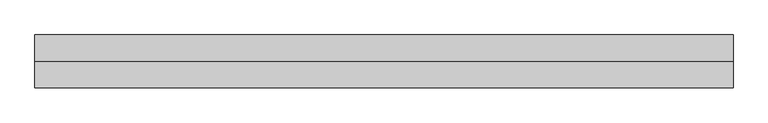
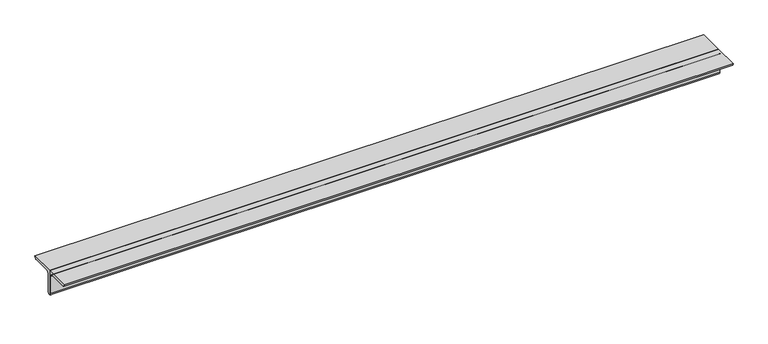
"""IFC4 building model written with IfcOpenShell, lengths in millimetres: member geometry, 0123_Steel Framing_2Ls-KSD3502 : H_SB_AR_S03_2Ls-130x130x12_HBR4."""

import ifcopenshell
import ifcopenshell.guid

model = None  # the IFC model being written
_history = None  # IfcOwnerHistory: only IFC2X3 demands one
_inside = {}  # id of a spatial element -> (the spatial element, [elements in it])
_under = {}  # id of a project, library or spatial element -> (it, [spatial elements below it])
_declared = {}  # id of a project -> (the project, [libraries it declares])
_typed = {}  # id of a type object -> (the type object, [elements of that type])
_made_of = {}  # id of a material, layer set ... -> (it, [elements and type objects made of it])


def new_model(schema):
    """Start an empty IFC model of exactly this schema.

    Asked for "IFC4X3", IfcOpenShell would pick the latest addendum, in which some entities
    have other attributes; the version numbers below select the first issue.
    IFC2X3 requires an IfcOwnerHistory on every rooted entity: one is made here for all.
    """
    global model, _history
    if schema == "IFC4X3":
        model = ifcopenshell.file(schema_version=(4, 3, 0, 0))
    else:
        model = ifcopenshell.file(schema=schema)
    _inside.clear()
    _under.clear()
    _declared.clear()
    _typed.clear()
    _made_of.clear()
    _history = None
    if model.schema == "IFC2X3":
        org = make("IfcOrganization", Name="unknown")
        user = make(
            "IfcPersonAndOrganization",
            ThePerson=make("IfcPerson", FamilyName="unknown"),
            TheOrganization=org,
        )
        app = make(
            "IfcApplication",
            ApplicationDeveloper=org,
            Version="unknown",
            ApplicationFullName="unknown",
            ApplicationIdentifier="unknown",
        )
        _history = make(
            "IfcOwnerHistory",
            OwningUser=user,
            OwningApplication=app,
            ChangeAction="ADDED",
            CreationDate=0,
        )
    return model


def make(cls, **values):
    """One entity of the class cls with the attributes given. An attribute that is None is left unset."""
    return model.create_entity(
        cls, **{name: value for name, value in values.items() if value is not None}
    )


def rooted(cls, **values):
    """An entity with a GlobalId (a new one), such as an element, a storey or a relation."""
    return make(cls, GlobalId=ifcopenshell.guid.new(), OwnerHistory=_history, **values)


def si_unit(unit_type, name, prefix=None):
    """IfcSIUnit, for example si_unit("LENGTHUNIT", "METRE", prefix="MILLI")."""
    return make("IfcSIUnit", UnitType=unit_type, Prefix=prefix, Name=name)


def assignment(units):
    """IfcUnitAssignment: the units of a project."""
    return None if units is None else make("IfcUnitAssignment", Units=units)


def point(xyz):
    """IfcCartesianPoint."""
    return None if xyz is None else make("IfcCartesianPoint", Coordinates=xyz)


def direction(xyz):
    """IfcDirection."""
    return None if xyz is None else make("IfcDirection", DirectionRatios=xyz)


def frame(location, z_axis=None, x_axis=None):
    """IfcAxis2Placement3D, a coordinate frame: its origin and axes. An axis left out is left unset."""
    return make(
        "IfcAxis2Placement3D",
        Location=point(location),
        Axis=direction(z_axis),
        RefDirection=direction(x_axis),
    )


def frame_2d(location, x_axis=None):
    """IfcAxis2Placement2D, a coordinate frame in the plane: its origin and x axis."""
    return make(
        "IfcAxis2Placement2D", Location=point(location), RefDirection=direction(x_axis)
    )


def origin():
    """The frame at (0, 0, 0) with its axes left unset."""
    return frame((0.0, 0.0, 0.0))


def place(relative_to, where):
    """IfcLocalPlacement: puts the frame where relative to a parent placement (None: the world)."""
    return make(
        "IfcLocalPlacement", PlacementRelTo=relative_to, RelativePlacement=where
    )


def context(
    kind, dimensions, precision=None, world=None, true_north=None, identifier=None
):
    """IfcGeometricRepresentationContext, for example the 3D "Model" context."""
    return make(
        "IfcGeometricRepresentationContext",
        ContextIdentifier=identifier,
        ContextType=kind,
        CoordinateSpaceDimension=dimensions,
        Precision=precision,
        WorldCoordinateSystem=world,
        TrueNorth=true_north,
    )


def project(units=None, contexts=None):
    """IfcProject with its units and contexts."""
    return rooted(
        "IfcProject",
        Name="project",
        RepresentationContexts=contexts,
        UnitsInContext=assignment(units),
    )


def spatial(cls, under=None, at=None, **own):
    """A site, building, storey or space (cls), placed at a placement, below another one or the project."""
    s = rooted(cls, ObjectPlacement=at, **own)
    if under is not None:
        _under.setdefault(under.id(), (under, []))[1].append(s)
    return s


def polyline(points):
    """IfcPolyline through the points."""
    return make("IfcPolyline", Points=[point(p) for p in points])


def circle_curve(where, radius):
    """IfcCircle in the frame where."""
    return make("IfcCircle", Position=where, Radius=radius)


def trimmed(basis, trim1, trim2, sense, master):
    """IfcTrimmedCurve: the piece of a basis curve between two trims."""
    return make(
        "IfcTrimmedCurve",
        BasisCurve=basis,
        Trim1=trim1,
        Trim2=trim2,
        SenseAgreement=sense,
        MasterRepresentation=master,
    )


def segment(curve, same_sense, transition):
    """IfcCompositeCurveSegment."""
    return make(
        "IfcCompositeCurveSegment",
        Transition=transition,
        SameSense=same_sense,
        ParentCurve=curve,
    )


def composite_curve(segments, self_intersect=None):
    """IfcCompositeCurve: segments joined end to end."""
    return make("IfcCompositeCurve", Segments=segments, SelfIntersect=self_intersect)


def outline(outer, holes=None, kind="AREA"):
    """IfcArbitraryClosedProfileDef: a profile drawn as a closed curve; with holes, ...WithVoids."""
    if holes is None:
        return make("IfcArbitraryClosedProfileDef", ProfileType=kind, OuterCurve=outer)
    return make(
        "IfcArbitraryProfileDefWithVoids",
        ProfileType=kind,
        OuterCurve=outer,
        InnerCurves=holes,
    )


def extrude(swept, where, along, depth):
    """IfcExtrudedAreaSolid: the profile swept, set in the frame where, extruded along a direction by depth."""
    return make(
        "IfcExtrudedAreaSolid",
        SweptArea=swept,
        Position=where,
        ExtrudedDirection=direction(along),
        Depth=depth,
    )


def shape(context_of_items, identifier, shape_type, items):
    """IfcShapeRepresentation: the items that make up one representation, for example the "Body"."""
    return make(
        "IfcShapeRepresentation",
        ContextOfItems=context_of_items,
        RepresentationIdentifier=identifier,
        RepresentationType=shape_type,
        Items=items,
    )


def source(mapping_origin, context_of_items, identifier, shape_type, items):
    """IfcRepresentationMap: a shape defined once, which mapped items show again and again."""
    return make(
        "IfcRepresentationMap",
        MappingOrigin=mapping_origin,
        MappedRepresentation=shape(context_of_items, identifier, shape_type, items),
    )


def transform(
    local_origin,
    x_axis=None,
    y_axis=None,
    z_axis=None,
    scale=None,
    scale2=None,
    scale3=None,
    uniform=True,
):
    """IfcCartesianTransformationOperator3D, or its non-uniform kind. x_axis, y_axis, z_axis: its Axis1, 2, 3."""
    if uniform:
        return make(
            "IfcCartesianTransformationOperator3D",
            Axis1=direction(x_axis),
            Axis2=direction(y_axis),
            LocalOrigin=point(local_origin),
            Scale=scale,
            Axis3=direction(z_axis),
        )
    return make(
        "IfcCartesianTransformationOperator3DnonUniform",
        Axis1=direction(x_axis),
        Axis2=direction(y_axis),
        LocalOrigin=point(local_origin),
        Scale=scale,
        Axis3=direction(z_axis),
        Scale2=scale2,
        Scale3=scale3,
    )


def mapped(mapping_source, mapping_target):
    """IfcMappedItem: shows the shape of a source again, moved by a transform."""
    return make(
        "IfcMappedItem", MappingSource=mapping_source, MappingTarget=mapping_target
    )


def made_of(thing, what):
    """Note that an element or type object is made of a material, layer set ...; save() writes the relation."""
    if what is not None:
        _made_of.setdefault(what.id(), (what, []))[1].append(thing)
    return thing


def element(
    cls,
    number,
    at=None,
    inside=None,
    cuts=None,
    type_object=None,
    material=None,
    context=None,
    identifier="Body",
    shape_type=None,
    held_by="IfcProductDefinitionShape",
    body=None,
    shapes=None,
    **own,
):
    """One element of the class cls, such as IfcWall. Its Tag is "e" and its number.

    at: its placement. inside: the storey or other place that contains it. cuts: it is an
    opening in that element (IfcRelVoidsElement). A single representation is given by context,
    identifier, shape_type and body (its items); several are given by shapes. held_by: the class
    of the entity that holds the representations. save() writes the other relations.
    """
    e = rooted(cls, Tag="e%d" % number, ObjectPlacement=at, **own)
    if body is not None:
        shapes = [shape(context, identifier, shape_type, body)]
    if shapes is not None:
        e.Representation = make(held_by, Representations=shapes)
    if inside is not None:
        _inside.setdefault(inside.id(), (inside, []))[1].append(e)
    if cuts is not None:
        rooted(
            "IfcRelVoidsElement", RelatingBuildingElement=cuts, RelatedOpeningElement=e
        )
    if type_object is not None:
        _typed.setdefault(type_object.id(), (type_object, []))[1].append(e)
    return made_of(e, material)


def aggregate(whole, parts):
    """IfcRelAggregates: a whole, such as a stair, and the parts it consists of."""
    return rooted("IfcRelAggregates", RelatingObject=whole, RelatedObjects=parts)


def save(model, path):
    """Write the relations noted so far, then the file.

    IfcRelAggregates (storeys below a building ...), IfcRelContainedInSpatialStructure (elements
    in a storey), IfcRelDefinesByType, IfcRelAssociatesMaterial and IfcRelDeclares: one each for
    every whole, place, type object, material and project.
    """
    for whole, parts in _under.values():
        aggregate(whole, parts)
    for where, things in _inside.values():
        rooted(
            "IfcRelContainedInSpatialStructure",
            RelatedElements=things,
            RelatingStructure=where,
        )
    for kind, things in _typed.values():
        rooted("IfcRelDefinesByType", RelatedObjects=things, RelatingType=kind)
    for what, things in _made_of.values():
        rooted("IfcRelAssociatesMaterial", RelatedObjects=things, RelatingMaterial=what)
    for by, libraries in _declared.values():
        rooted("IfcRelDeclares", RelatingContext=by, RelatedDefinitions=libraries)
    model.write(path)


def member_9e88965d(model_context):
    return source(origin(), model_context, "Body", "SweptSolid", [
        extrude(outline(composite_curve([segment(polyline([(0.0, 36.4), (130.0, 36.4)]), True, "CONTINUOUS"), segment(trimmed(circle_curve(frame_2d((118.0, 36.4)), 12.0), [point((130.0, 36.4))], [point((118.0, 24.4))], False, "CARTESIAN"), True, "CONTINUOUS"), segment(polyline([(118.0, 24.4), (24.0, 24.4)]), True, "CONTINUOUS"), segment(trimmed(circle_curve(frame_2d((24.0, 12.4)), 12.0), [point((24.0, 24.4))], [point((12.0, 12.4))], True, "CARTESIAN"), True, "CONTINUOUS"), segment(polyline([(12.0, 12.4), (12.0, -81.6)]), True, "CONTINUOUS"), segment(trimmed(circle_curve(frame_2d((0.0, -81.6)), 12.0), [point((12.0, -81.6))], [point((0.0, -93.6))], False, "CARTESIAN"), True, "CONTINUOUS"), segment(polyline([(0.0, -93.6), (0.0, 36.4)]), True, "CONTINUOUS")], self_intersect=False)), frame((-1720.2330278, 0.0, 0.0), z_axis=(1.0, 0.0, 0.0), x_axis=(0.0, 1.0, 0.0)), (0.0, 0.0, 1.0), 3440.4660555),
        extrude(outline(composite_curve([segment(polyline([(0.0, 36.4), (0.0, -93.6)]), True, "CONTINUOUS"), segment(trimmed(circle_curve(frame_2d((0.0, -81.6)), 12.0), [point((0.0, -93.6))], [point((-12.0, -81.6))], False, "CARTESIAN"), True, "CONTINUOUS"), segment(polyline([(-12.0, -81.6), (-12.0, 12.4)]), True, "CONTINUOUS"), segment(trimmed(circle_curve(frame_2d((-24.0, 12.4)), 12.0), [point((-12.0, 12.4))], [point((-24.0, 24.4))], True, "CARTESIAN"), True, "CONTINUOUS"), segment(polyline([(-24.0, 24.4), (-118.0, 24.4)]), True, "CONTINUOUS"), segment(trimmed(circle_curve(frame_2d((-118.0, 36.4)), 12.0), [point((-118.0, 24.4))], [point((-130.0, 36.4))], False, "CARTESIAN"), True, "CONTINUOUS"), segment(polyline([(-130.0, 36.4), (0.0, 36.4)]), True, "CONTINUOUS")], self_intersect=False)), frame((-1720.2330278, 0.0, 0.0), z_axis=(1.0, 0.0, 0.0), x_axis=(0.0, 1.0, 0.0)), (0.0, 0.0, 1.0), 3440.4660555),
    ])


if __name__ == "__main__":
    model = new_model("IFC4")
    model_context = context("Model", 3, world=origin())
    ifc_project = project(units=[si_unit("LENGTHUNIT", "METRE", prefix="MILLI")], contexts=[model_context])
    site = spatial("IfcSite", under=ifc_project)
    building = spatial("IfcBuilding", under=site)
    placement = place(None, origin())
    member_shape = member_9e88965d(model_context)
    element("IfcMember", 1, ObjectType="0123_Steel Framing_2Ls-KSD3502 : H_SB_AR_S03_2Ls-130x130x12_HBR4", at=placement, inside=building, context=model_context, shape_type="MappedRepresentation", body=[
        mapped(member_shape, transform((0.0, 0.0, 0.0), x_axis=(1.0, 0.0, 0.0), y_axis=(0.0, 1.0, 0.0), z_axis=(0.0, 0.0, 1.0))),
    ])
    save(model, "model.ifc")

# Revit data of these elements
# Type "0123_Steel Framing_2Ls-KSD3502 : H_SB_AR_S03_2Ls-130x130x12_HBR4"
#   Assembly Code = "B10"
#   Legs = "SLBB"
#   W = 8.97
#   Perimeter = 1.04 m²/m
#   Nominal Weight = 46.80 kgf/m
#   Length [instance default] = 1000 mm
#   Space = 0 mm
#   b = 130 mm
#   d = 130 mm
#   t = 12 mm
#   y = 36.4 mm
#   A = 0.005952 m²
#   Structural Material [instance default] = Steel ASTM A36
# Element 1 (IfcMember, "0123_Steel Framing_2Ls-KSD3502 : H_SB_AR_S03_2Ls-130x130x12_HBR4")
#   Structural Material = Steel, 45-345
#   Materials on its faces: "Steel, 45-345"
# Materials
#   "Steel ASTM A36": class "Metal", colour RGB 199 199 199, transparency 0, Description = "Structural steel, ASTM A36 Grade B, mill finish", Cost = 0
#   "Steel, 45-345": class "Metal", colour RGB 189 187 185, transparency 0, Description = "Steel 345 MPa", Cost = 0
